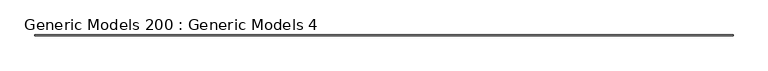
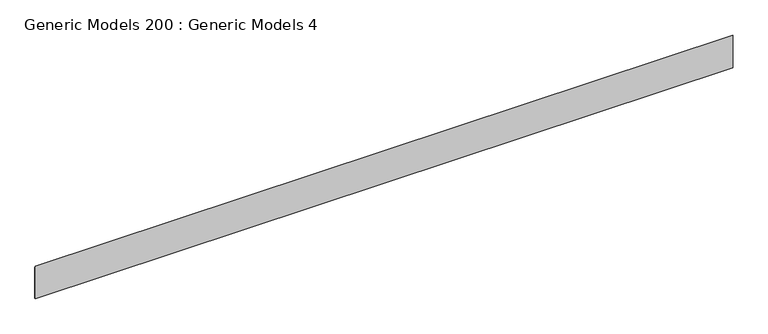
"""IFC4 building model written with IfcOpenShell, lengths in millimetres: proxy geometry, Generic Models 200 : Generic Models 4."""

from ifc_helpers import new_model, si_unit, frame, origin, place, context, project, spatial, polyline, outline, extrude, source, transform, mapped, element, save


def generic_models_200_generic_models_4_64e646ec(model_context):
    return source(origin(), model_context, "Body", "SweptSolid", [
        extrude(outline(polyline([(-5651.7555338, 126343.791), (-5669.5355338, 126343.791), (-5669.5355338, 126953.2066323), (-5651.7555338, 126918.5824217), (-5651.7555338, 126343.791)])), frame((-10259.9171316, 0.0, 0.0), z_axis=(1.0, 0.0, 0.0), x_axis=(0.0, 1.0, 0.0)), (0.0, 0.0, 1.0), 12456.843502),
    ])


if __name__ == "__main__":
    model = new_model("IFC4")
    model_context = context("Model", 3, world=origin())
    ifc_project = project(units=[si_unit("LENGTHUNIT", "METRE", prefix="MILLI")], contexts=[model_context])
    site = spatial("IfcSite", under=ifc_project)
    building = spatial("IfcBuilding", under=site)
    placement = place(None, origin())
    generic_models_200_generic_models_4_shape = generic_models_200_generic_models_4_64e646ec(model_context)
    element("IfcBuildingElementProxy", 1, Name="Generic Models 200 : Generic Models 4", ObjectType="Generic Models 200 : Generic Models 4", at=placement, inside=building, context=model_context, shape_type="MappedRepresentation", body=[
        mapped(generic_models_200_generic_models_4_shape, transform((0.0, 0.0, 0.0), x_axis=(1.0, 0.0, 0.0), y_axis=(0.0, 1.0, 0.0), z_axis=(0.0, 0.0, 1.0))),
    ])
    save(model, "model.ifc")

# Revit data of these elements
# Element 1 (IfcBuildingElementProxy, "Generic Models 200 : Generic Models 4")
#   Materials on its faces: "_7/8\" SMOOTH TROWEL EXTERIOR STUCCO (COLOR PER OWNER)"
# Materials
#   "_7/8\" SMOOTH TROWEL EXTERIOR STUCCO (COLOR PER OWNER)": class "Generic", colour RGB 233 233 233, transparency 0, Cost = 0
